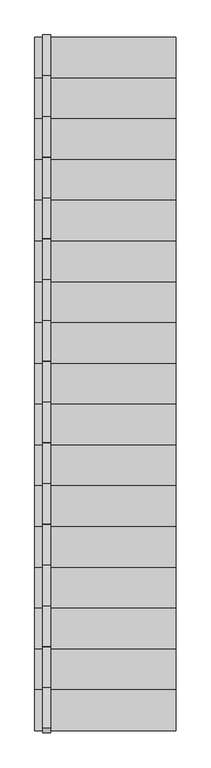
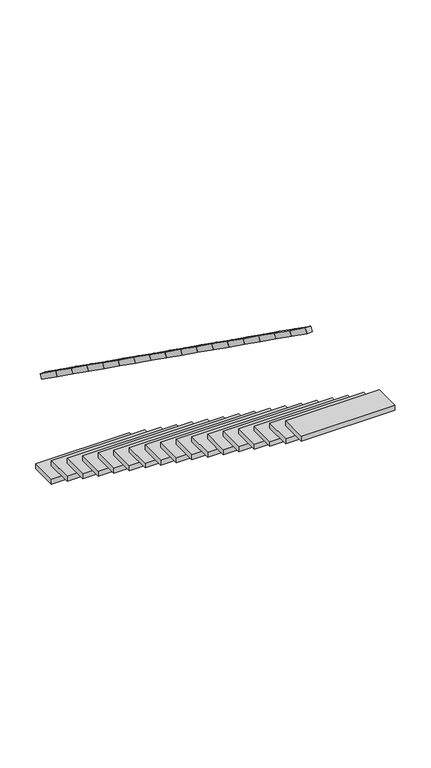
"""IFC4 building model written with IfcOpenShell, lengths in millimetres: stair geometry,   92587 :   92587."""

import ifcopenshell
import ifcopenshell.guid

model = None  # the IFC model being written
_history = None  # IfcOwnerHistory: only IFC2X3 demands one
_inside = {}  # id of a spatial element -> (the spatial element, [elements in it])
_under = {}  # id of a project, library or spatial element -> (it, [spatial elements below it])
_declared = {}  # id of a project -> (the project, [libraries it declares])
_typed = {}  # id of a type object -> (the type object, [elements of that type])
_made_of = {}  # id of a material, layer set ... -> (it, [elements and type objects made of it])


def new_model(schema):
    """Start an empty IFC model of exactly this schema.

    Asked for "IFC4X3", IfcOpenShell would pick the latest addendum, in which some entities
    have other attributes; the version numbers below select the first issue.
    IFC2X3 requires an IfcOwnerHistory on every rooted entity: one is made here for all.
    """
    global model, _history
    if schema == "IFC4X3":
        model = ifcopenshell.file(schema_version=(4, 3, 0, 0))
    else:
        model = ifcopenshell.file(schema=schema)
    _inside.clear()
    _under.clear()
    _declared.clear()
    _typed.clear()
    _made_of.clear()
    _history = None
    if model.schema == "IFC2X3":
        org = make("IfcOrganization", Name="unknown")
        user = make(
            "IfcPersonAndOrganization",
            ThePerson=make("IfcPerson", FamilyName="unknown"),
            TheOrganization=org,
        )
        app = make(
            "IfcApplication",
            ApplicationDeveloper=org,
            Version="unknown",
            ApplicationFullName="unknown",
            ApplicationIdentifier="unknown",
        )
        _history = make(
            "IfcOwnerHistory",
            OwningUser=user,
            OwningApplication=app,
            ChangeAction="ADDED",
            CreationDate=0,
        )
    return model


def make(cls, **values):
    """One entity of the class cls with the attributes given. An attribute that is None is left unset."""
    return model.create_entity(
        cls, **{name: value for name, value in values.items() if value is not None}
    )


def rooted(cls, **values):
    """An entity with a GlobalId (a new one), such as an element, a storey or a relation."""
    return make(cls, GlobalId=ifcopenshell.guid.new(), OwnerHistory=_history, **values)


def si_unit(unit_type, name, prefix=None):
    """IfcSIUnit, for example si_unit("LENGTHUNIT", "METRE", prefix="MILLI")."""
    return make("IfcSIUnit", UnitType=unit_type, Prefix=prefix, Name=name)


def assignment(units):
    """IfcUnitAssignment: the units of a project."""
    return None if units is None else make("IfcUnitAssignment", Units=units)


def point(xyz):
    """IfcCartesianPoint."""
    return None if xyz is None else make("IfcCartesianPoint", Coordinates=xyz)


def direction(xyz):
    """IfcDirection."""
    return None if xyz is None else make("IfcDirection", DirectionRatios=xyz)


def frame(location, z_axis=None, x_axis=None):
    """IfcAxis2Placement3D, a coordinate frame: its origin and axes. An axis left out is left unset."""
    return make(
        "IfcAxis2Placement3D",
        Location=point(location),
        Axis=direction(z_axis),
        RefDirection=direction(x_axis),
    )


def origin():
    """The frame at (0, 0, 0) with its axes left unset."""
    return frame((0.0, 0.0, 0.0))


def place(relative_to, where):
    """IfcLocalPlacement: puts the frame where relative to a parent placement (None: the world)."""
    return make(
        "IfcLocalPlacement", PlacementRelTo=relative_to, RelativePlacement=where
    )


def context(
    kind, dimensions, precision=None, world=None, true_north=None, identifier=None
):
    """IfcGeometricRepresentationContext, for example the 3D "Model" context."""
    return make(
        "IfcGeometricRepresentationContext",
        ContextIdentifier=identifier,
        ContextType=kind,
        CoordinateSpaceDimension=dimensions,
        Precision=precision,
        WorldCoordinateSystem=world,
        TrueNorth=true_north,
    )


def project(units=None, contexts=None):
    """IfcProject with its units and contexts."""
    return rooted(
        "IfcProject",
        Name="project",
        RepresentationContexts=contexts,
        UnitsInContext=assignment(units),
    )


def spatial(cls, under=None, at=None, **own):
    """A site, building, storey or space (cls), placed at a placement, below another one or the project."""
    s = rooted(cls, ObjectPlacement=at, **own)
    if under is not None:
        _under.setdefault(under.id(), (under, []))[1].append(s)
    return s


def polyline(points):
    """IfcPolyline through the points."""
    return make("IfcPolyline", Points=[point(p) for p in points])


def outline(outer, holes=None, kind="AREA"):
    """IfcArbitraryClosedProfileDef: a profile drawn as a closed curve; with holes, ...WithVoids."""
    if holes is None:
        return make("IfcArbitraryClosedProfileDef", ProfileType=kind, OuterCurve=outer)
    return make(
        "IfcArbitraryProfileDefWithVoids",
        ProfileType=kind,
        OuterCurve=outer,
        InnerCurves=holes,
    )


def extrude(swept, where, along, depth):
    """IfcExtrudedAreaSolid: the profile swept, set in the frame where, extruded along a direction by depth."""
    return make(
        "IfcExtrudedAreaSolid",
        SweptArea=swept,
        Position=where,
        ExtrudedDirection=direction(along),
        Depth=depth,
    )


def shape(context_of_items, identifier, shape_type, items):
    """IfcShapeRepresentation: the items that make up one representation, for example the "Body"."""
    return make(
        "IfcShapeRepresentation",
        ContextOfItems=context_of_items,
        RepresentationIdentifier=identifier,
        RepresentationType=shape_type,
        Items=items,
    )


def source(mapping_origin, context_of_items, identifier, shape_type, items):
    """IfcRepresentationMap: a shape defined once, which mapped items show again and again."""
    return make(
        "IfcRepresentationMap",
        MappingOrigin=mapping_origin,
        MappedRepresentation=shape(context_of_items, identifier, shape_type, items),
    )


def transform(
    local_origin,
    x_axis=None,
    y_axis=None,
    z_axis=None,
    scale=None,
    scale2=None,
    scale3=None,
    uniform=True,
):
    """IfcCartesianTransformationOperator3D, or its non-uniform kind. x_axis, y_axis, z_axis: its Axis1, 2, 3."""
    if uniform:
        return make(
            "IfcCartesianTransformationOperator3D",
            Axis1=direction(x_axis),
            Axis2=direction(y_axis),
            LocalOrigin=point(local_origin),
            Scale=scale,
            Axis3=direction(z_axis),
        )
    return make(
        "IfcCartesianTransformationOperator3DnonUniform",
        Axis1=direction(x_axis),
        Axis2=direction(y_axis),
        LocalOrigin=point(local_origin),
        Scale=scale,
        Axis3=direction(z_axis),
        Scale2=scale2,
        Scale3=scale3,
    )


def mapped(mapping_source, mapping_target):
    """IfcMappedItem: shows the shape of a source again, moved by a transform."""
    return make(
        "IfcMappedItem", MappingSource=mapping_source, MappingTarget=mapping_target
    )


def made_of(thing, what):
    """Note that an element or type object is made of a material, layer set ...; save() writes the relation."""
    if what is not None:
        _made_of.setdefault(what.id(), (what, []))[1].append(thing)
    return thing


def element(
    cls,
    number,
    at=None,
    inside=None,
    cuts=None,
    type_object=None,
    material=None,
    context=None,
    identifier="Body",
    shape_type=None,
    held_by="IfcProductDefinitionShape",
    body=None,
    shapes=None,
    **own,
):
    """One element of the class cls, such as IfcWall. Its Tag is "e" and its number.

    at: its placement. inside: the storey or other place that contains it. cuts: it is an
    opening in that element (IfcRelVoidsElement). A single representation is given by context,
    identifier, shape_type and body (its items); several are given by shapes. held_by: the class
    of the entity that holds the representations. save() writes the other relations.
    """
    e = rooted(cls, Tag="e%d" % number, ObjectPlacement=at, **own)
    if body is not None:
        shapes = [shape(context, identifier, shape_type, body)]
    if shapes is not None:
        e.Representation = make(held_by, Representations=shapes)
    if inside is not None:
        _inside.setdefault(inside.id(), (inside, []))[1].append(e)
    if cuts is not None:
        rooted(
            "IfcRelVoidsElement", RelatingBuildingElement=cuts, RelatedOpeningElement=e
        )
    if type_object is not None:
        _typed.setdefault(type_object.id(), (type_object, []))[1].append(e)
    return made_of(e, material)


def aggregate(whole, parts):
    """IfcRelAggregates: a whole, such as a stair, and the parts it consists of."""
    return rooted("IfcRelAggregates", RelatingObject=whole, RelatedObjects=parts)


def save(model, path):
    """Write the relations noted so far, then the file.

    IfcRelAggregates (storeys below a building ...), IfcRelContainedInSpatialStructure (elements
    in a storey), IfcRelDefinesByType, IfcRelAssociatesMaterial and IfcRelDeclares: one each for
    every whole, place, type object, material and project.
    """
    for whole, parts in _under.values():
        aggregate(whole, parts)
    for where, things in _inside.values():
        rooted(
            "IfcRelContainedInSpatialStructure",
            RelatedElements=things,
            RelatingStructure=where,
        )
    for kind, things in _typed.values():
        rooted("IfcRelDefinesByType", RelatedObjects=things, RelatingType=kind)
    for what, things in _made_of.values():
        rooted("IfcRelAssociatesMaterial", RelatedObjects=things, RelatingMaterial=what)
    for by, libraries in _declared.values():
        rooted("IfcRelDeclares", RelatingContext=by, RelatedDefinitions=libraries)
    model.write(path)


def stair_667f7fc2(model_context):
    return source(origin(), model_context, "Body", "SweptSolid", [
        extrude(outline(polyline([(0.0, -319.1002977), (0.0, 0.0), (50.0, 0.0), (50.0, -319.1002977), (0.0, -319.1002977)])), frame((162072.7593015, 34520.3024209, 4178.947508), z_axis=(0.0, 0.5797550216229128, 0.8147908411997622), x_axis=(-1.0, 0.0, 0.0)), (0.0, 0.0, 1.0), 50.0),
        extrude(outline(polyline([(0.0, -319.1002977), (0.0, 0.0), (50.0, 0.0), (50.0, -319.1002977), (0.0, -319.1002977)])), frame((162072.7593015, 34780.3024209, 3993.947508), z_axis=(0.0, 0.5797550216229022, 0.8147908411997696), x_axis=(-1.0, 0.0, 0.0)), (0.0, 0.0, 1.0), 50.0),
        extrude(outline(polyline([(0.0, -319.1002977), (0.0, 0.0), (50.0, 0.0), (50.0, -319.1002977), (0.0, -319.1002977)])), frame((162072.7593015, 35040.3024209, 3808.947508), z_axis=(0.0, 0.5797550216229116, 0.814790841199763), x_axis=(-1.0, 0.0, 0.0)), (0.0, 0.0, 1.0), 50.0),
        extrude(outline(polyline([(0.0, -319.1002977), (0.0, 0.0), (50.0, 0.0), (50.0, -319.1002977), (0.0, -319.1002977)])), frame((162072.7593015, 35300.3024209, 3623.947508), z_axis=(0.0, 0.5797550216229086, 0.8147908411997651), x_axis=(-1.0, 0.0, 0.0)), (0.0, 0.0, 1.0), 50.0),
        extrude(outline(polyline([(0.0, -319.1002977), (0.0, 0.0), (50.0, 0.0), (50.0, -319.1002977), (0.0, -319.1002977)])), frame((162072.7593015, 35560.3024209, 3438.947508), z_axis=(0.0, 0.5797550216229094, 0.8147908411997645), x_axis=(-1.0, 0.0, 0.0)), (0.0, 0.0, 1.0), 50.0),
        extrude(outline(polyline([(0.0, -319.1002977), (0.0, 0.0), (50.0, 0.0), (50.0, -319.1002977), (0.0, -319.1002977)])), frame((162072.7593015, 35820.3024209, 3253.947508), z_axis=(0.0, 0.5797550216228999, 0.8147908411997712), x_axis=(-1.0, 0.0, 0.0)), (0.0, 0.0, 1.0), 50.0),
        extrude(outline(polyline([(0.0, -319.1002977), (0.0, 0.0), (50.0, 0.0), (50.0, -319.1002977), (0.0, -319.1002977)])), frame((162072.7593015, 36080.3024209, 3068.947508), z_axis=(0.0, 0.579755021622915, 0.8147908411997605), x_axis=(-1.0, 0.0, 0.0)), (0.0, 0.0, 1.0), 50.0),
        extrude(outline(polyline([(0.0, -319.1002977), (0.0, 0.0), (50.0, 0.0), (50.0, -319.1002977), (0.0, -319.1002977)])), frame((162072.7593015, 36340.3024209, 2883.947508), z_axis=(0.0, 0.5797550216229139, 0.8147908411997614), x_axis=(-1.0, 0.0, 0.0)), (0.0, 0.0, 1.0), 50.0),
        extrude(outline(polyline([(0.0, -319.1002977), (0.0, 0.0), (50.0, 0.0), (50.0, -319.1002977), (0.0, -319.1002977)])), frame((162072.7593015, 36600.3024209, 2698.947508), z_axis=(0.0, 0.5797550216229128, 0.8147908411997622), x_axis=(-1.0, 0.0, 0.0)), (0.0, 0.0, 1.0), 50.0),
        extrude(outline(polyline([(0.0, -319.1002977), (0.0, 0.0), (50.0, 0.0), (50.0, -319.1002977), (0.0, -319.1002977)])), frame((162072.7593015, 36860.3024209, 2513.947508), z_axis=(0.0, 0.5797550216228966, 0.8147908411997736), x_axis=(-1.0, 0.0, 0.0)), (0.0, 0.0, 1.0), 50.0),
        extrude(outline(polyline([(0.0, -319.1002977), (0.0, 0.0), (50.0, 0.0), (50.0, -319.1002977), (0.0, -319.1002977)])), frame((162072.7593015, 37120.3024209, 2328.947508), z_axis=(0.0, 0.5797550216229123, 0.8147908411997625), x_axis=(-1.0, 0.0, 0.0)), (0.0, 0.0, 1.0), 50.0),
        extrude(outline(polyline([(0.0, -319.1002977), (0.0, 0.0), (50.0, 0.0), (50.0, -319.1002977), (0.0, -319.1002977)])), frame((162072.7593015, 37380.3024209, 2143.947508), z_axis=(0.0, 0.5797550216229139, 0.8147908411997614), x_axis=(-1.0, 0.0, 0.0)), (0.0, 0.0, 1.0), 50.0),
        extrude(outline(polyline([(0.0, -319.1002977), (0.0, 0.0), (50.0, 0.0), (50.0, -319.1002977), (0.0, -319.1002977)])), frame((162072.7593015, 37640.3024209, 1958.947508), z_axis=(0.0, 0.5797550216228999, 0.8147908411997712), x_axis=(-1.0, 0.0, 0.0)), (0.0, 0.0, 1.0), 50.0),
        extrude(outline(polyline([(0.0, -319.1002977), (0.0, 0.0), (50.0, 0.0), (50.0, -319.1002977), (0.0, -319.1002977)])), frame((162072.7593015, 37900.3024209, 1773.947508), z_axis=(0.0, 0.579755021622915, 0.8147908411997605), x_axis=(-1.0, 0.0, 0.0)), (0.0, 0.0, 1.0), 50.0),
        extrude(outline(polyline([(0.0, -319.1002977), (0.0, 0.0), (50.0, 0.0), (50.0, -319.1002977), (0.0, -319.1002977)])), frame((162072.7593015, 38160.3024209, 1588.947508), z_axis=(0.0, 0.579755021622908, 0.8147908411997654), x_axis=(-1.0, 0.0, 0.0)), (0.0, 0.0, 1.0), 50.0),
        extrude(outline(polyline([(0.0, -319.1002977), (0.0, 0.0), (50.0, 0.0), (50.0, -319.1002977), (0.0, -319.1002977)])), frame((162072.7593015, 38420.3024209, 1403.947508), z_axis=(0.0, 0.5797550216229066, 0.8147908411997665), x_axis=(-1.0, 0.0, 0.0)), (0.0, 0.0, 1.0), 50.0),
        extrude(outline(polyline([(0.0, -319.1002977), (0.0, 0.0), (50.0, 0.0), (50.0, -319.1002977), (0.0, -319.1002977)])), frame((162072.7593015, 38680.3024209, 1218.947508), z_axis=(0.0, 0.5797550216228985, 0.8147908411997723), x_axis=(-1.0, 0.0, 0.0)), (0.0, 0.0, 1.0), 50.0),
        extrude(outline(polyline([(161972.7593015, 38694.7962965), (161972.7593015, 38954.7962965), (162872.7593015, 38954.7962965), (162872.7593015, 38694.7962965), (161972.7593015, 38694.7962965)])), frame((0.0, 0.0, 135.0), z_axis=(0.0, 0.0, 1.0), x_axis=(1.0, 0.0, 0.0)), (0.0, 0.0, 1.0), 50.0),
        extrude(outline(polyline([(161972.7593015, 38434.7962965), (161972.7593015, 38694.7962965), (162872.7593015, 38694.7962965), (162872.7593015, 38434.7962965), (161972.7593015, 38434.7962965)])), frame((0.0, 0.0, 320.0), z_axis=(0.0, 0.0, 1.0), x_axis=(1.0, 0.0, 0.0)), (0.0, 0.0, 1.0), 50.0),
        extrude(outline(polyline([(161972.7593015, 38174.7962965), (161972.7593015, 38434.7962965), (162872.7593015, 38434.7962965), (162872.7593015, 38174.7962965), (161972.7593015, 38174.7962965)])), frame((0.0, 0.0, 505.0), z_axis=(0.0, 0.0, 1.0), x_axis=(1.0, 0.0, 0.0)), (0.0, 0.0, 1.0), 50.0),
        extrude(outline(polyline([(161972.7593015, 37914.7962965), (161972.7593015, 38174.7962965), (162872.7593015, 38174.7962965), (162872.7593015, 37914.7962965), (161972.7593015, 37914.7962965)])), frame((0.0, 0.0, 690.0), z_axis=(0.0, 0.0, 1.0), x_axis=(1.0, 0.0, 0.0)), (0.0, 0.0, 1.0), 50.0),
        extrude(outline(polyline([(161972.7593015, 37654.7962965), (161972.7593015, 37914.7962965), (162872.7593015, 37914.7962965), (162872.7593015, 37654.7962965), (161972.7593015, 37654.7962965)])), frame((0.0, 0.0, 875.0), z_axis=(0.0, 0.0, 1.0), x_axis=(1.0, 0.0, 0.0)), (0.0, 0.0, 1.0), 50.0),
        extrude(outline(polyline([(161972.7593015, 37394.7962965), (161972.7593015, 37654.7962965), (162872.7593015, 37654.7962965), (162872.7593015, 37394.7962965), (161972.7593015, 37394.7962965)])), frame((0.0, 0.0, 1060.0), z_axis=(0.0, 0.0, 1.0), x_axis=(1.0, 0.0, 0.0)), (0.0, 0.0, 1.0), 50.0),
        extrude(outline(polyline([(161972.7593015, 37134.7962965), (161972.7593015, 37394.7962965), (162872.7593015, 37394.7962965), (162872.7593015, 37134.7962965), (161972.7593015, 37134.7962965)])), frame((0.0, 0.0, 1245.0), z_axis=(0.0, 0.0, 1.0), x_axis=(1.0, 0.0, 0.0)), (0.0, 0.0, 1.0), 50.0),
        extrude(outline(polyline([(161972.7593015, 36874.7962965), (161972.7593015, 37134.7962965), (162872.7593015, 37134.7962965), (162872.7593015, 36874.7962965), (161972.7593015, 36874.7962965)])), frame((0.0, 0.0, 1430.0), z_axis=(0.0, 0.0, 1.0), x_axis=(1.0, 0.0, 0.0)), (0.0, 0.0, 1.0), 50.0),
        extrude(outline(polyline([(161972.7593015, 36614.7962965), (161972.7593015, 36874.7962965), (162872.7593015, 36874.7962965), (162872.7593015, 36614.7962965), (161972.7593015, 36614.7962965)])), frame((0.0, 0.0, 1615.0), z_axis=(0.0, 0.0, 1.0), x_axis=(1.0, 0.0, 0.0)), (0.0, 0.0, 1.0), 50.0),
        extrude(outline(polyline([(161972.7593015, 36354.7962965), (161972.7593015, 36614.7962965), (162872.7593015, 36614.7962965), (162872.7593015, 36354.7962965), (161972.7593015, 36354.7962965)])), frame((0.0, 0.0, 1800.0), z_axis=(0.0, 0.0, 1.0), x_axis=(1.0, 0.0, 0.0)), (0.0, 0.0, 1.0), 50.0),
        extrude(outline(polyline([(161972.7593015, 36094.7962965), (161972.7593015, 36354.7962965), (162872.7593015, 36354.7962965), (162872.7593015, 36094.7962965), (161972.7593015, 36094.7962965)])), frame((0.0, 0.0, 1985.0), z_axis=(0.0, 0.0, 1.0), x_axis=(1.0, 0.0, 0.0)), (0.0, 0.0, 1.0), 50.0),
        extrude(outline(polyline([(161972.7593015, 35834.7962965), (161972.7593015, 36094.7962965), (162872.7593015, 36094.7962965), (162872.7593015, 35834.7962965), (161972.7593015, 35834.7962965)])), frame((0.0, 0.0, 2170.0), z_axis=(0.0, 0.0, 1.0), x_axis=(1.0, 0.0, 0.0)), (0.0, 0.0, 1.0), 50.0),
        extrude(outline(polyline([(161972.7593015, 35574.7962965), (161972.7593015, 35834.7962965), (162872.7593015, 35834.7962965), (162872.7593015, 35574.7962965), (161972.7593015, 35574.7962965)])), frame((0.0, 0.0, 2355.0), z_axis=(0.0, 0.0, 1.0), x_axis=(1.0, 0.0, 0.0)), (0.0, 0.0, 1.0), 50.0),
        extrude(outline(polyline([(161972.7593015, 35314.7962965), (161972.7593015, 35574.7962965), (162872.7593015, 35574.7962965), (162872.7593015, 35314.7962965), (161972.7593015, 35314.7962965)])), frame((0.0, 0.0, 2540.0), z_axis=(0.0, 0.0, 1.0), x_axis=(1.0, 0.0, 0.0)), (0.0, 0.0, 1.0), 50.0),
        extrude(outline(polyline([(161972.7593015, 35054.7962965), (161972.7593015, 35314.7962965), (162872.7593015, 35314.7962965), (162872.7593015, 35054.7962965), (161972.7593015, 35054.7962965)])), frame((0.0, 0.0, 2725.0), z_axis=(0.0, 0.0, 1.0), x_axis=(1.0, 0.0, 0.0)), (0.0, 0.0, 1.0), 50.0),
        extrude(outline(polyline([(161972.7593015, 34794.7962965), (161972.7593015, 35054.7962965), (162872.7593015, 35054.7962965), (162872.7593015, 34794.7962965), (161972.7593015, 34794.7962965)])), frame((0.0, 0.0, 2910.0), z_axis=(0.0, 0.0, 1.0), x_axis=(1.0, 0.0, 0.0)), (0.0, 0.0, 1.0), 50.0),
        extrude(outline(polyline([(161972.7593015, 34534.7962965), (161972.7593015, 34794.7962965), (162872.7593015, 34794.7962965), (162872.7593015, 34534.7962965), (161972.7593015, 34534.7962965)])), frame((0.0, 0.0, 3095.0), z_axis=(0.0, 0.0, 1.0), x_axis=(1.0, 0.0, 0.0)), (0.0, 0.0, 1.0), 50.0),
    ])


if __name__ == "__main__":
    model = new_model("IFC4")
    model_context = context("Model", 3, world=origin())
    ifc_project = project(units=[si_unit("LENGTHUNIT", "METRE", prefix="MILLI")], contexts=[model_context])
    site = spatial("IfcSite", under=ifc_project)
    building = spatial("IfcBuilding", under=site)
    placement = place(None, origin())
    stair_shape = stair_667f7fc2(model_context)
    element("IfcStair", 1, ObjectType="  92587 :   92587", at=placement, inside=building, context=model_context, shape_type="MappedRepresentation", body=[
        mapped(stair_shape, transform((0.0, 0.0, 0.0), x_axis=(1.0, 0.0, 0.0), y_axis=(0.0, 1.0, 0.0), z_axis=(0.0, 0.0, 1.0))),
    ])
    save(model, "model.ifc")

# Revit data of these elements
# Type "  92587 :   92587"
#   Abrechnungsart = "St"
#   Allright_Bauteil_ID = "0121Tre0785067483"
#   Material = "Stahlbeton"
#   Objektname = "Treppe"
#   NameOverride = " "
#   ThermalTransmittance = 0.0000 BTU/(h·ft²·°F)
#   NosingLength = 0.000 m
#   NumberOfRiser = 18
#   NumberOfTreads = 17
#   RiserHeight = 1.850 m
#   TreadLength = 2.600 m
#   IsExternal = no
#   FireExit = no
#   HandicapAccessible = no
#   HasNonSkidSurface = no
# Element 1 (IfcStair, "  92587 :   92587")
#   Materials on its faces: "*1", "weiss"
# Materials
#   "*1": class "Unassigned", colour RGB 175 175 175, transparency 0
#   "weiss": class "Unassigned", colour RGB 255 255 255, transparency 0
